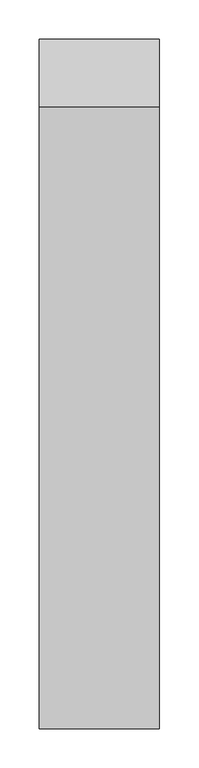
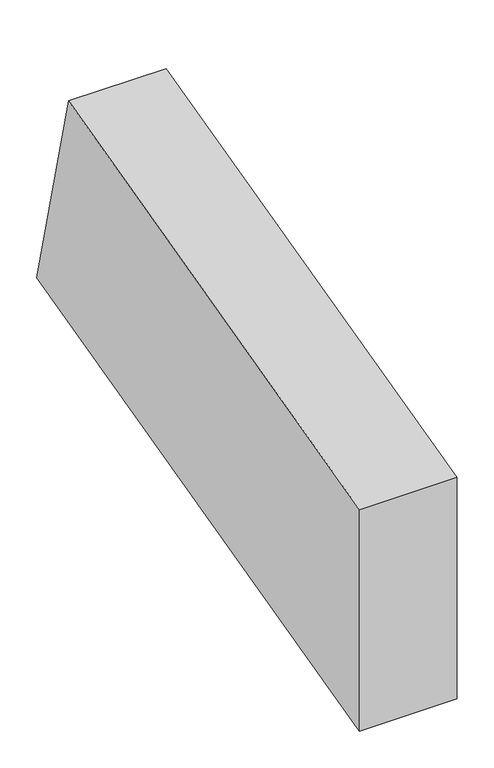
"""IFC4 building model written with IfcOpenShell, lengths in millimetres: proxy geometry, Framing016 3117 : Framing016 3117."""

from ifc_helpers import new_model, si_unit, frame, origin, place, context, project, spatial, polyline, outline, extrude, source, transform, mapped, element, save


def generic_models_47f04879(model_context):
    return source(origin(), model_context, "Body", "SweptSolid", [
        extrude(outline(polyline([(8857.883325, 43384.4932401), (9647.0095123, 43581.9371332), (9733.2922309, 43237.0426118), (8857.883325, 43018.0404079), (8857.883325, 43384.4932401)])), frame((5541.8883192, 0.0, 0.0), z_axis=(1.0, 0.0, 0.0), x_axis=(0.0, 1.0, 0.0)), (0.0, 0.0, 1.0), 152.4),
    ])


if __name__ == "__main__":
    model = new_model("IFC4")
    model_context = context("Model", 3, world=origin())
    ifc_project = project(units=[si_unit("LENGTHUNIT", "METRE", prefix="MILLI")], contexts=[model_context])
    site = spatial("IfcSite", under=ifc_project)
    building = spatial("IfcBuilding", under=site)
    placement = place(None, origin())
    generic_models_shape = generic_models_47f04879(model_context)
    element("IfcBuildingElementProxy", 1, Name="Framing016 3117 : Framing016 3117", ObjectType="Framing016 3117 : Framing016 3117", at=placement, inside=building, context=model_context, shape_type="MappedRepresentation", body=[
        mapped(generic_models_shape, transform((0.0, 0.0, 0.0), x_axis=(1.0, 0.0, 0.0), y_axis=(0.0, 1.0, 0.0), z_axis=(0.0, 0.0, 1.0))),
    ])
    save(model, "model.ifc")

# Revit data of these elements
# Type "Framing016 3117 : Framing016 3117"
#   NameOverride = "Framing016"
# Element 1 (IfcBuildingElementProxy, "Framing016 3117 : Framing016 3117")
#   Materials on its faces: "WOOD FRAMING (SEE STRUCT DWGS)"
# Materials
#   "WOOD FRAMING (SEE STRUCT DWGS)": class "Unassigned", colour RGB 224 188 168, transparency 0, Cost = 0
